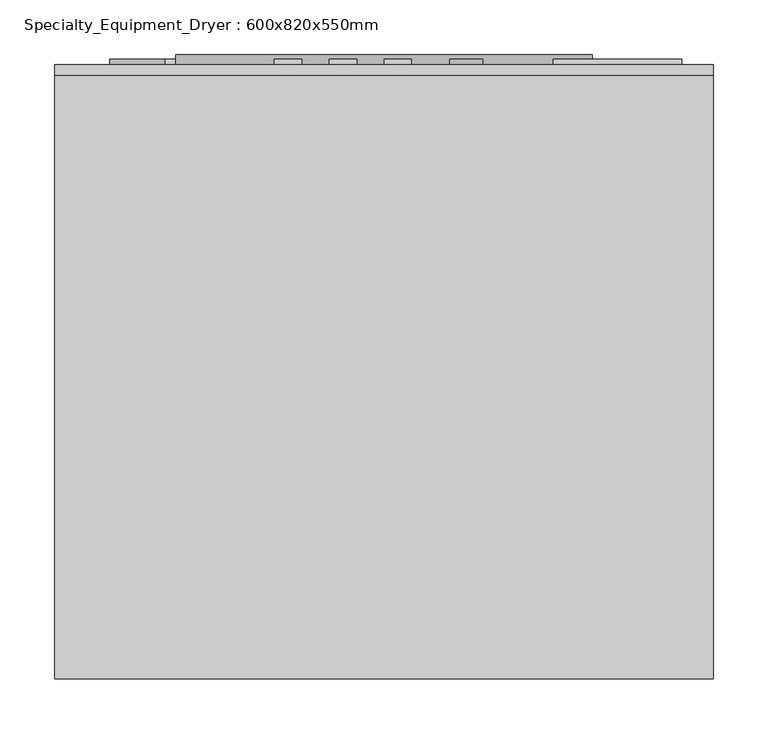
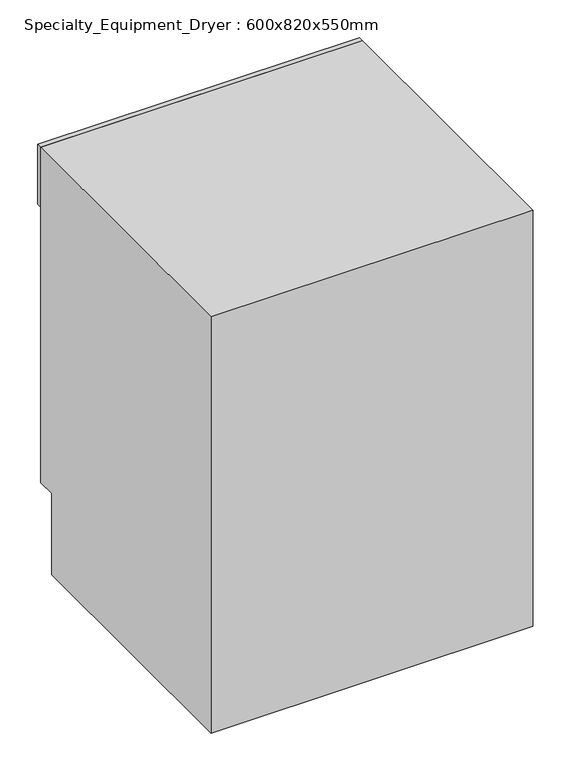
"""IFC4 building model written with IfcOpenShell, lengths in millimetres: proxy geometry, Specialty_Equipment_Dryer : 600x820x550mm."""

from ifc_helpers import new_model, si_unit, point, frame, frame_2d, origin, place, context, project, spatial, polyline, circle_curve, trimmed, segment, composite_curve, outline, extrude, source, transform, mapped, element, save
from ifc_brep_helpers import plane_surface, revolved_surface, advanced_brep


def specialty_equipment_dryer_600x820x550mm_3611e1b7(model_context):
    return source(origin(), model_context, "Body", "SolidModel", [
        advanced_brep(
        [(-451.3135585, 212.25, 0.0), (-451.3135585, 212.25, 820.0), (-451.3135585, 762.25, 820.0), (-451.3135585, 762.25, 160.0), (-451.3135585, 727.25, 160.0), (-451.3135585, 727.25, 0.0), (148.6864415, 212.25, 0.0), (148.6864415, 727.25, 0.0), (148.6864415, 727.25, 160.0), (148.6864415, 762.25, 160.0), (148.6864415, 762.25, 820.0), (148.6864415, 212.25, 820.0), (38.6864415, 762.25, 440.0), (-341.3135585, 762.25, 440.0), (38.6864415, 512.25, 440.0), (-341.3135585, 512.25, 440.0)],
        [
            (0, 1),
            (1, 2),
            (2, 3),
            (3, 4),
            (4, 5),
            (5, 0),
            (6, 7),
            (7, 8),
            (8, 9),
            (9, 10),
            (10, 11),
            (11, 6),
            (0, 6),
            (11, 1),
            (10, 2),
            (9, 3),
            (12, 13, circle_curve(frame((-151.3135585, 762.25, 440.0), z_axis=(0.0, -1.0, 0.0), x_axis=(-1.0, 0.0, 0.0)), 190.0)),
            (13, 12, circle_curve(frame((-151.3135585, 762.25, 440.0), z_axis=(0.0, -1.0, 0.0), x_axis=(-1.0, 0.0, 0.0)), 190.0)),
            (8, 4),
            (7, 5),
            (14, 15, circle_curve(frame((-151.3135585, 512.25, 440.0), z_axis=(0.0, 1.0, 0.0), x_axis=(-1.0, 0.0, 0.0)), 190.0)),
            (15, 14, circle_curve(frame((-151.3135585, 512.25, 440.0), z_axis=(0.0, 1.0, 0.0), x_axis=(-1.0, 0.0, 0.0)), 190.0)),
            (15, 13),
            (12, 14),
        ],
        [
            plane_surface(frame((-451.3135585, 212.25, 820.0), z_axis=(-1.0, 0.0, 0.0), x_axis=(0.0, 0.0, 1.0))),
            plane_surface(frame((148.6864415, 212.25, 820.0), z_axis=(1.0, 0.0, 0.0), x_axis=(0.0, 0.0, -1.0))),
            plane_surface(frame((-451.3135585, 212.25, 0.0), z_axis=(0.0, -1.0, 0.0), x_axis=(1.0, 0.0, 0.0))),
            plane_surface(frame((-451.3135585, 212.25, 820.0), z_axis=(0.0, 0.0, 1.0), x_axis=(1.0, 0.0, 0.0))),
            plane_surface(frame((-451.3135585, 762.25, 820.0), z_axis=(0.0, 1.0, 0.0), x_axis=(1.0, 0.0, 0.0))),
            plane_surface(frame((-451.3135585, 762.25, 160.0), z_axis=(0.0, 0.0, -1.0), x_axis=(1.0, 0.0, 0.0))),
            plane_surface(frame((-451.3135585, 727.25, 160.0), z_axis=(0.0, 1.0, 0.0), x_axis=(1.0, 0.0, 0.0))),
            plane_surface(frame((-451.3135585, 727.25, 0.0), z_axis=(0.0, 0.0, -1.0), x_axis=(1.0, 0.0, 0.0))),
            plane_surface(frame((-341.3135585, 512.25, 440.0), z_axis=(0.0, 1.0, 0.0), x_axis=(0.0, 0.0, -1.0))),
            revolved_surface(polyline([(-341.3135585, 512.25, 440.0), (-341.3135585, 762.25, 440.0)]), (-151.3135585, 762.25, 440.0), (0.0, -1.0, 0.0)),
        ],
        [
            (0, [[1, 2, 3, 4, 5, 6]]),
            (1, [[7, 8, 9, 10, 11, 12]]),
            (2, [[-1, 13, -12, 14]]),
            (3, [[-2, -14, -11, 15]]),
            (4, [[-3, -15, -10, 16], [17, 18]]),
            (5, [[-4, -16, -9, 19]]),
            (6, [[-5, -19, -8, 20]]),
            (7, [[-6, -20, -7, -13]]),
            (8, [[21, 22]]),
            (9, [[-22, 23, -17, 24]]),
            (9, [[-21, -24, -18, -23]]),
        ],
    ),
        extrude(outline(polyline([(3.1591715, 777.25), (119.995263, 777.25), (119.995263, 772.25), (3.1591715, 772.25), (3.1591715, 777.25)])), frame((0.0, 0.0, 736.0845617), z_axis=(0.0, 0.0, 1.0), x_axis=(1.0, 0.0, 0.0)), (0.0, 0.0, 1.0), 25.0),
        extrude(outline(polyline([(-251.3135585, 777.25), (-226.3135585, 777.25), (-226.3135585, 772.25), (-251.3135585, 772.25), (-251.3135585, 777.25)])), frame((0.0, 0.0, 741.0845617), z_axis=(0.0, 0.0, 1.0), x_axis=(1.0, 0.0, 0.0)), (0.0, 0.0, 1.0), 40.0),
        extrude(outline(composite_curve([segment(trimmed(circle_curve(frame_2d((761.0845617, -376.3135585)), 25.0), [point((761.0845617, -401.3135585))], [point((761.0845617, -351.3135585))], False, "CARTESIAN"), True, "CONTINUOUS"), segment(trimmed(circle_curve(frame_2d((761.0845617, -376.3135585)), 25.0), [point((761.0845617, -351.3135585))], [point((761.0845617, -401.3135585))], False, "CARTESIAN"), True, "CONTINUOUS")], self_intersect=False)), frame((0.0, 772.25, 0.0), z_axis=(0.0, 1.0, 0.0), x_axis=(0.0, 0.0, 1.0)), (0.0, 0.0, 1.0), 5.0),
        extrude(outline(composite_curve([segment(trimmed(circle_curve(frame_2d((761.0845617, -76.3135585)), 15.0), [point((761.0845617, -91.3135585))], [point((761.0845617, -61.3135585))], False, "CARTESIAN"), True, "CONTINUOUS"), segment(trimmed(circle_curve(frame_2d((761.0845617, -76.3135585)), 15.0), [point((761.0845617, -61.3135585))], [point((761.0845617, -91.3135585))], False, "CARTESIAN"), True, "CONTINUOUS")], self_intersect=False)), frame((0.0, 772.25, 0.0), z_axis=(0.0, 1.0, 0.0), x_axis=(0.0, 0.0, 1.0)), (0.0, 0.0, 1.0), 5.0),
        extrude(outline(polyline([(-392.6202937, 777.25), (-323.3523296, 777.25), (-323.3523296, 772.25), (-392.6202937, 772.25), (-392.6202937, 777.25)])), frame((0.0, 0.0, 209.0795094), z_axis=(0.0, 0.0, 1.0), x_axis=(1.0, 0.0, 0.0)), (0.0, 0.0, 1.0), 10.0),
        extrude(outline(polyline([(-151.3135585, 777.25), (-126.3135585, 777.25), (-126.3135585, 772.25), (-151.3135585, 772.25), (-151.3135585, 777.25)])), frame((0.0, 0.0, 741.0845617), z_axis=(0.0, 0.0, 1.0), x_axis=(1.0, 0.0, 0.0)), (0.0, 0.0, 1.0), 40.0),
        extrude(outline(polyline([(-201.3135585, 777.25), (-176.3135585, 777.25), (-176.3135585, 772.25), (-201.3135585, 772.25), (-201.3135585, 777.25)])), frame((0.0, 0.0, 741.0845617), z_axis=(0.0, 0.0, 1.0), x_axis=(1.0, 0.0, 0.0)), (0.0, 0.0, 1.0), 40.0),
        extrude(outline(polyline([(-451.3135585, 772.25), (148.6864415, 772.25), (148.6864415, 762.25), (-451.3135585, 762.25), (-451.3135585, 772.25)])), frame((0.0, 0.0, 702.1691233), z_axis=(0.0, 0.0, 1.0), x_axis=(1.0, 0.0, 0.0)), (0.0, 0.0, 1.0), 117.8308767),
        extrude(outline(composite_curve([segment(trimmed(circle_curve(frame_2d((214.7704069, -357.8865689)), 35.0), [point((214.7704069, -392.8865689))], [point((214.7704069, -322.8865689))], False, "CARTESIAN"), True, "CONTINUOUS"), segment(trimmed(circle_curve(frame_2d((214.7704069, -357.8865689)), 35.0), [point((214.7704069, -322.8865689))], [point((214.7704069, -392.8865689))], False, "CARTESIAN"), True, "CONTINUOUS")], self_intersect=False)), frame((0.0, 762.25, 0.0), z_axis=(0.0, 1.0, 0.0), x_axis=(0.0, 0.0, 1.0)), (0.0, 0.0, 1.0), 10.0),
        extrude(outline(composite_curve([segment(trimmed(circle_curve(frame_2d((440.0, -151.3135585)), 190.0), [point((440.0, -341.3135585))], [point((440.0, 38.6864415))], False, "CARTESIAN"), True, "CONTINUOUS"), segment(trimmed(circle_curve(frame_2d((440.0, -151.3135585)), 190.0), [point((440.0, 38.6864415))], [point((440.0, -341.3135585))], False, "CARTESIAN"), True, "CONTINUOUS")], self_intersect=False), holes=[composite_curve([segment(trimmed(circle_curve(frame_2d((440.0, -151.3135585)), 140.0), [point((440.0, -291.3135585))], [point((440.0, -11.3135585))], True, "CARTESIAN"), True, "CONTINUOUS"), segment(trimmed(circle_curve(frame_2d((440.0, -151.3135585)), 140.0), [point((440.0, -11.3135585))], [point((440.0, -291.3135585))], True, "CARTESIAN"), True, "CONTINUOUS")], self_intersect=False)]), frame((0.0, 762.25, 0.0), z_axis=(0.0, 1.0, 0.0), x_axis=(0.0, 0.0, 1.0)), (0.0, 0.0, 1.0), 19.0),
    ])


if __name__ == "__main__":
    model = new_model("IFC4")
    model_context = context("Model", 3, world=origin())
    ifc_project = project(units=[si_unit("LENGTHUNIT", "METRE", prefix="MILLI")], contexts=[model_context])
    site = spatial("IfcSite", under=ifc_project)
    building = spatial("IfcBuilding", under=site)
    placement = place(None, origin())
    specialty_equipment_dryer_600x820x550mm_shape = specialty_equipment_dryer_600x820x550mm_3611e1b7(model_context)
    element("IfcBuildingElementProxy", 1, Name="Specialty_Equipment_Dryer : 600x820x550mm", ObjectType="Specialty_Equipment_Dryer : 600x820x550mm", at=placement, inside=building, context=model_context, shape_type="MappedRepresentation", body=[
        mapped(specialty_equipment_dryer_600x820x550mm_shape, transform((0.0, 0.0, 0.0), x_axis=(1.0, 0.0, 0.0), y_axis=(0.0, 1.0, 0.0), z_axis=(0.0, 0.0, 1.0))),
    ])
    save(model, "model.ifc")

# Revit data of these elements
# Type "Specialty_Equipment_Dryer : 600x820x550mm"
#   Label = "D"
#   Keynote = "N"
#   Depth = 550 mm
#   Height = 820 mm
#   Plinth Depth = 35 mm
#   Plinth Height = 160 mm
#   Width = 600 mm
#   Material = Metal - Paint Finish - Ivory, Glossy
# Element 1 (IfcBuildingElementProxy, "Specialty_Equipment_Dryer : 600x820x550mm")
#   Materials on its faces: "Plastic - Black", "Metal - Stainless Steel", "Metal - Paint Finish - Ivory, Glossy"
# Materials
#   "Metal - Paint Finish - Ivory, Glossy": class "Paint", colour RGB 247 247 239, transparency 0
#   "Plastic - Black": class "Plastic", colour RGB 0 0 0, transparency 0.7
#   "Metal - Stainless Steel": class "Metal", colour RGB 57 57 57, transparency 0
